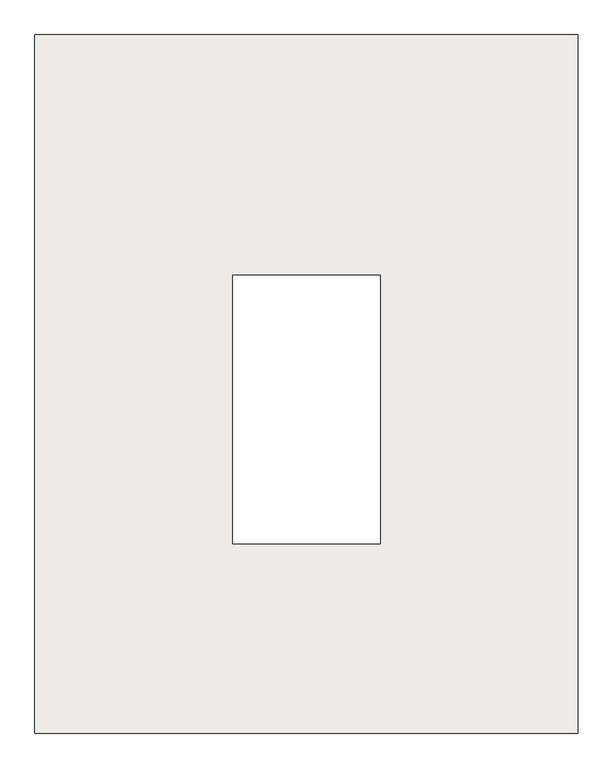
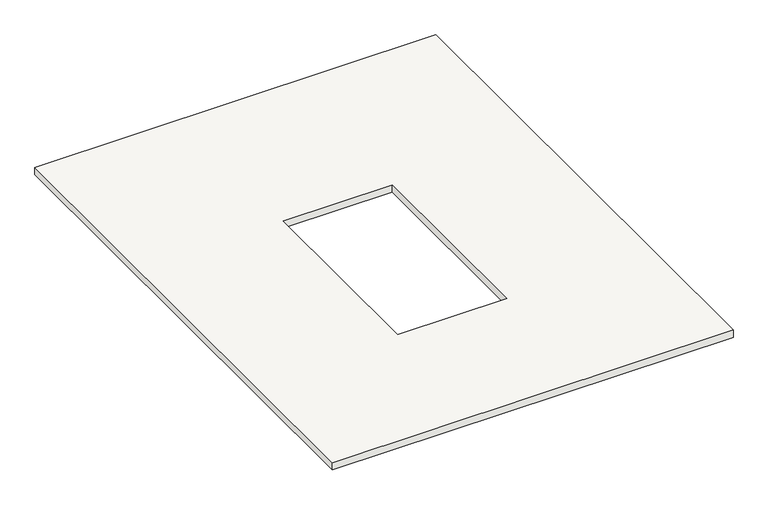
"""IFC4 building model written with IfcOpenShell, lengths in millimetres: slab geometry, Holzdecke."""

from ifc_helpers import new_model, si_unit, origin, origin_with_axes, place, context, project, spatial, polyline, outline, extrude, source, transform, mapped, element, save


def slab_db95388b(model_context):
    return source(origin(), model_context, "Body", "SweptSolid", [
        extrude(outline(polyline([(14000.0, 18002.8619019), (14000.0, 0.0), (0.0, 0.0), (0.0, 18002.8619019), (14000.0, 18002.8619019)]), holes=[polyline([(5100.0, 11802.8619019), (5100.0, 4877.8619019), (8900.0, 4877.8619019), (8900.0, 11802.8619019), (5100.0, 11802.8619019)])]), origin_with_axes(), (0.0, 0.0, 1.0), 270.0),
    ])


if __name__ == "__main__":
    model = new_model("IFC4")
    model_context = context("Model", 3, world=origin())
    ifc_project = project(units=[si_unit("LENGTHUNIT", "METRE", prefix="MILLI")], contexts=[model_context])
    site = spatial("IfcSite", under=ifc_project)
    building = spatial("IfcBuilding", under=site)
    placement = place(None, origin())
    slab_shape = slab_db95388b(model_context)
    element("IfcSlab", 1, ObjectType="Holzdecke", at=placement, inside=building, context=model_context, shape_type="MappedRepresentation", body=[
        mapped(slab_shape, transform((0.0, 0.0, 0.0), x_axis=(1.0, 0.0, 0.0), y_axis=(0.0, 1.0, 0.0), z_axis=(0.0, 0.0, 1.0))),
    ])
    save(model, "model.ifc")

# Revit data of these elements
# Element 1 (IfcSlab, "Holzdecke")
#   Materials on its faces: "holzschalung"
# Materials
#   "holzschalung": class "Unassigned", colour RGB 128 128 128, transparency 0
